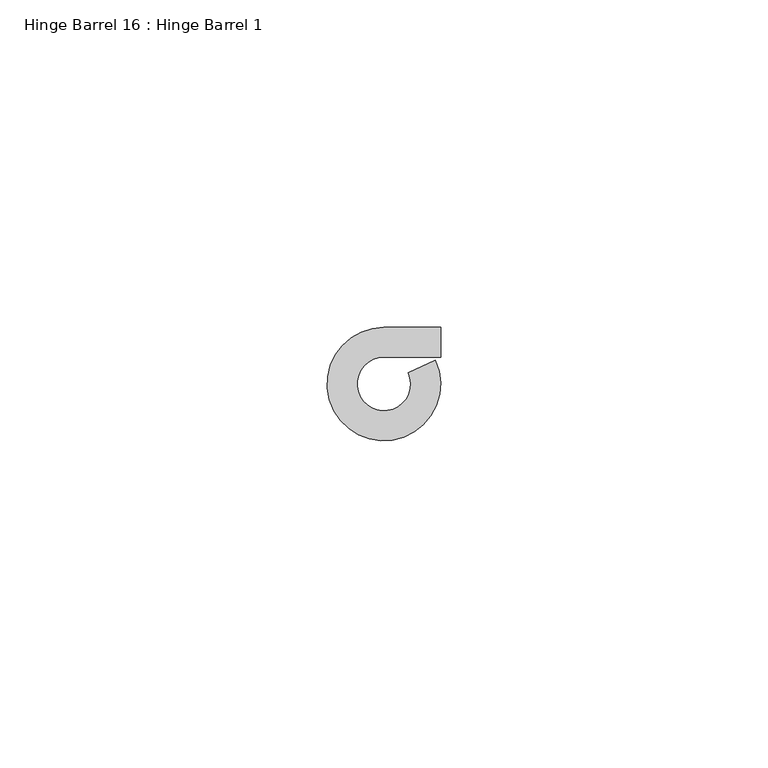
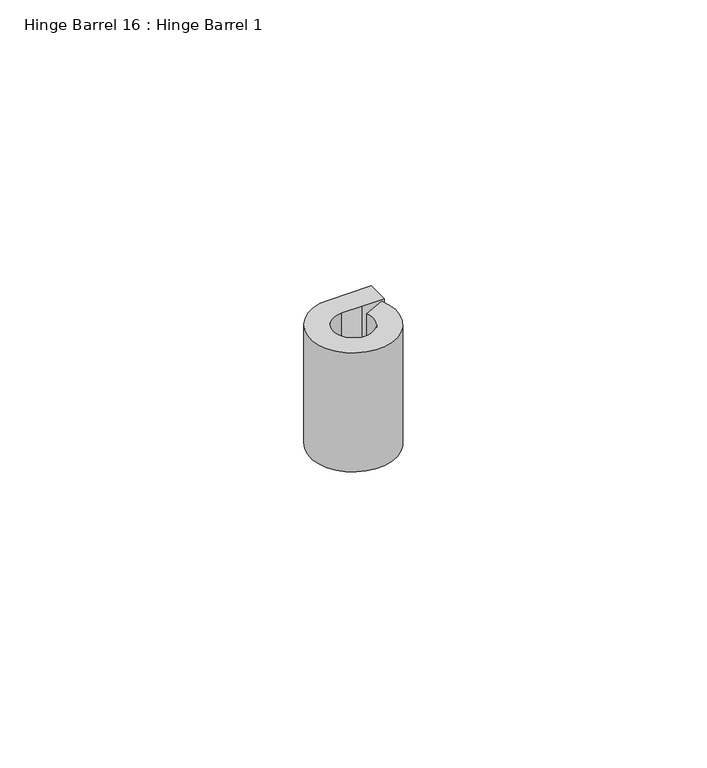
"""IFC4 building model written with IfcOpenShell, lengths in millimetres: proxy geometry, Hinge Barrel 16 : Hinge Barrel 1."""

from ifc_helpers import new_model, si_unit, point, frame, frame_2d, origin, place, context, project, spatial, polyline, circle_curve, trimmed, segment, composite_curve, outline, extrude, source, transform, mapped, element, save


def hinge_barrel_16_hinge_barrel_1_a937cab9(model_context):
    return source(origin(), model_context, "Body", "SweptSolid", [
        extrude(outline(composite_curve([segment(polyline([(587323.2214739, -533980.5883841), (587319.1320739, -533980.5883841)]), True, "CONTINUOUS"), segment(trimmed(circle_curve(frame_2d((587319.1320739, -533984.6777841)), 4.0894), [point((587319.1320739, -533980.5883841))], [point((587322.8436736, -533982.9610371))], True, "CARTESIAN"), True, "CONTINUOUS"), segment(polyline([(587322.8436736, -533982.9610371), (587326.986084, -533981.0450249)]), True, "CONTINUOUS"), segment(trimmed(circle_curve(frame_2d((587319.1320739, -533984.6777841)), 8.6534625), [point((587326.986084, -533981.0450249))], [point((587319.1320739, -533976.0243216))], False, "CARTESIAN"), True, "CONTINUOUS"), segment(polyline([(587319.1320739, -533976.0243216), (587327.7934739, -533976.0243216), (587327.7934739, -533980.5883841), (587323.2214739, -533980.5883841)]), True, "CONTINUOUS")], self_intersect=False)), frame((0.0, 0.0, 412.75), z_axis=(0.0, 0.0, 1.0), x_axis=(1.0, 0.0, 0.0)), (0.0, 0.0, 1.0), 25.4),
    ])


if __name__ == "__main__":
    model = new_model("IFC4")
    model_context = context("Model", 3, world=origin())
    ifc_project = project(units=[si_unit("LENGTHUNIT", "METRE", prefix="MILLI")], contexts=[model_context])
    site = spatial("IfcSite", under=ifc_project)
    building = spatial("IfcBuilding", under=site)
    placement = place(None, origin())
    hinge_barrel_16_hinge_barrel_1_shape = hinge_barrel_16_hinge_barrel_1_a937cab9(model_context)
    element("IfcBuildingElementProxy", 1, Name="Hinge Barrel 16 : Hinge Barrel 1", ObjectType="Hinge Barrel 16 : Hinge Barrel 1", at=placement, inside=building, context=model_context, shape_type="MappedRepresentation", body=[
        mapped(hinge_barrel_16_hinge_barrel_1_shape, transform((0.0, 0.0, 0.0), x_axis=(1.0, 0.0, 0.0), y_axis=(0.0, 1.0, 0.0), z_axis=(0.0, 0.0, 1.0))),
    ])
    save(model, "model.ifc")

# Revit data of these elements
# Element 1 (IfcBuildingElementProxy, "Hinge Barrel 16 : Hinge Barrel 1")
#   Materials on its faces: "6\"X6\" WELD-ON STL BUTT HINGE"
# Materials
#   "6\"X6\" WELD-ON STL BUTT HINGE": class "Metal", colour RGB 189 187 185, transparency 0, Description = "Carbon steel", Cost = 0
